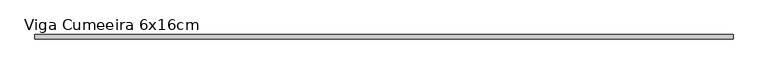
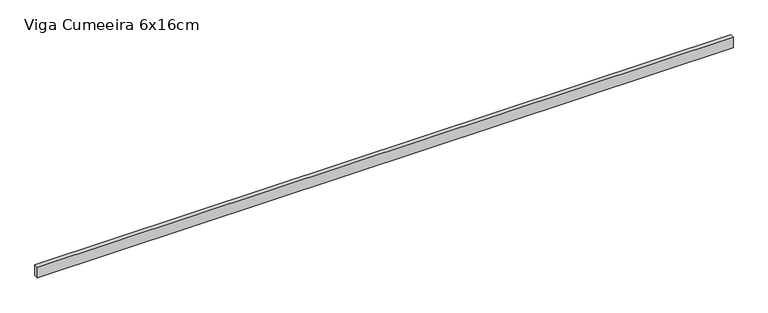
"""IFC4 building model written with IfcOpenShell, lengths in millimetres: beam geometry, Madeira de lei : Viga Cumeeira 6x16cm."""

from ifc_helpers import new_model, si_unit, frame, origin, place, context, project, spatial, polyline, outline, extrude, source, transform, mapped, element, save


def viga_cumeeira_6x16cm_10b61863(model_context):
    return source(origin(), model_context, "Body", "SweptSolid", [
        extrude(outline(polyline([(4969.4999994, 30.0), (4969.4999994, -30.0), (-4969.4999994, -30.0), (-4969.4999994, 30.0), (4969.4999994, 30.0)])), frame((0.0, 0.0, -80.0), z_axis=(0.0, 0.0, 1.0), x_axis=(1.0, 0.0, 0.0)), (0.0, 0.0, 1.0), 160.0),
    ])


if __name__ == "__main__":
    model = new_model("IFC4")
    model_context = context("Model", 3, world=origin())
    ifc_project = project(units=[si_unit("LENGTHUNIT", "METRE", prefix="MILLI")], contexts=[model_context])
    site = spatial("IfcSite", under=ifc_project)
    building = spatial("IfcBuilding", under=site)
    placement = place(None, origin())
    viga_cumeeira_6x16cm_shape = viga_cumeeira_6x16cm_10b61863(model_context)
    element("IfcBeam", 1, ObjectType="Madeira de lei : Viga Cumeeira 6x16cm", at=placement, inside=building, context=model_context, shape_type="MappedRepresentation", body=[
        mapped(viga_cumeeira_6x16cm_shape, transform((0.0, 0.0, 0.0), x_axis=(1.0, 0.0, 0.0), y_axis=(0.0, 1.0, 0.0), z_axis=(0.0, 0.0, 1.0))),
    ])
    save(model, "model.ifc")

# Revit data of these elements
# Type "Madeira de lei : Viga Cumeeira 6x16cm"
#   A = 0.02 m²
#   Length [instance default] = 1.524 m
#   b = 0.06 m
#   d = 0.16 m
#   Structural Material [instance default] = none
#   Assembly Code = ""
# Element 1 (IfcBeam, "Madeira de lei : Viga Cumeeira 6x16cm")
#   Structural Material = .MADEIRAMENTO
#   Materials on its faces: ".MADEIRAMENTO"
# Materials
#   ".MADEIRAMENTO": class ".CC_MADEIRAS", colour RGB 212 179 113, transparency 0, Cost = 0
